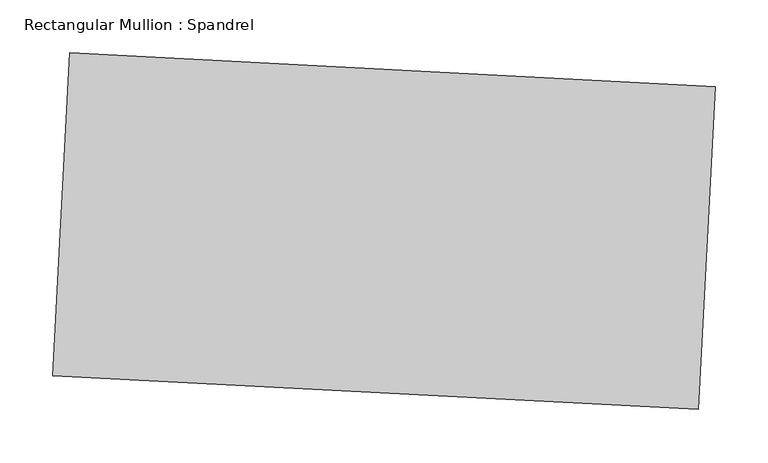
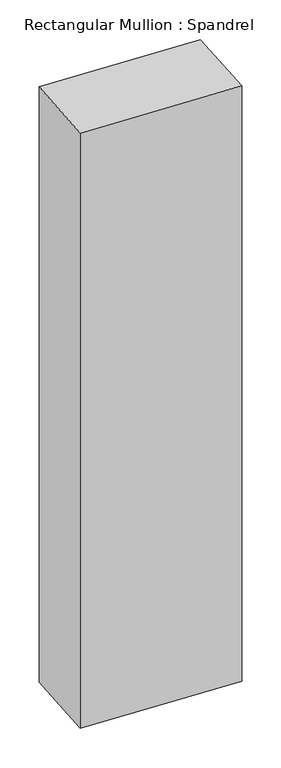
"""IFC4 building model written with IfcOpenShell, lengths in millimetres: member geometry, Rectangular Mullion : Spandrel."""

from ifc_helpers import new_model, si_unit, frame, origin, place, context, project, spatial, polyline, outline, extrude, source, transform, mapped, element, save


def rectangular_mullion_spandrel_10a84132(model_context):
    return source(origin(), model_context, "Body", "SweptSolid", [
        extrude(outline(polyline([(312.3582819, 136.2391416), (296.4062825, -168.1431406), (-312.3582819, -136.2391416), (-296.4062825, 168.1431406), (312.3582819, 136.2391416)])), frame((0.0, 0.0, -2445.9256159), z_axis=(0.0, 0.0, 1.0), x_axis=(1.0, 0.0, 0.0)), (0.0, 0.0, 1.0), 2445.9256159),
    ])


if __name__ == "__main__":
    model = new_model("IFC4")
    model_context = context("Model", 3, world=origin())
    ifc_project = project(units=[si_unit("LENGTHUNIT", "METRE", prefix="MILLI")], contexts=[model_context])
    site = spatial("IfcSite", under=ifc_project)
    building = spatial("IfcBuilding", under=site)
    placement = place(None, origin())
    rectangular_mullion_spandrel_shape = rectangular_mullion_spandrel_10a84132(model_context)
    element("IfcMember", 1, ObjectType="Rectangular Mullion : Spandrel", at=placement, inside=building, context=model_context, shape_type="MappedRepresentation", body=[
        mapped(rectangular_mullion_spandrel_shape, transform((0.0, 0.0, 0.0), x_axis=(1.0, 0.0, 0.0), y_axis=(0.0, 1.0, 0.0), z_axis=(0.0, 0.0, 1.0))),
    ])
    save(model, "model.ifc")

# Revit data of these elements
# Type "Rectangular Mullion : Spandrel"
#   built-in parameter 1007304 = 1 (stored number, unit not read)
#   built-in parameter 1007301 = 1 (stored number, unit not read)
#   built-in parameter 1007300 = 1 (stored number, unit not read)
# Element 1 (IfcMember, "Rectangular Mullion : Spandrel")
#   Materials on its faces: "Aluminum"
# Materials
#   "Aluminum": class "Metal", colour RGB 247 247 247, transparency 0, Description = "Aluminum 6061", Cost = 0
